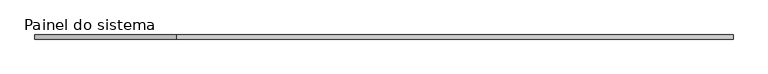
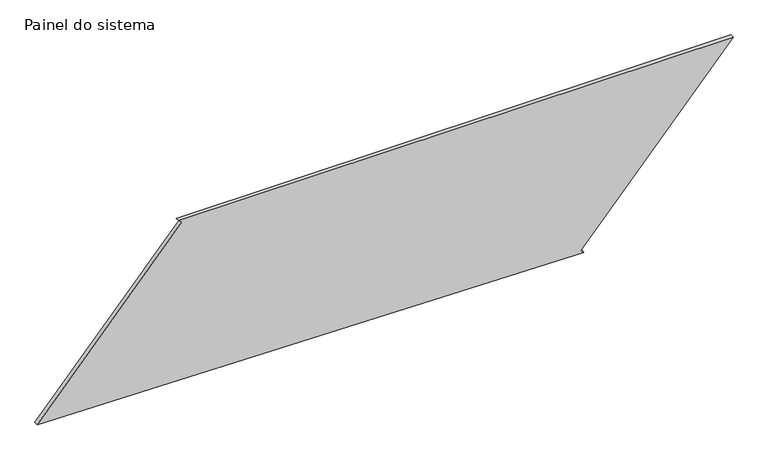
"""IFC4 building model written with IfcOpenShell, lengths in millimetres: plate geometry, Painel do sistema : Envidraçado."""

from ifc_helpers import new_model, si_unit, frame, origin, place, context, project, spatial, polyline, outline, extrude, source, transform, mapped, element, save


def painel_do_sistema_9e2e3e45(model_context):
    return source(origin(), model_context, "Body", "SweptSolid", [
        extrude(outline(polyline([(0.0, 1217.150078), (16.5356636, 1198.3998293), (1073.9840407, 2130.9533607), (1073.9840407, -1265.8401605), (1057.4483771, -1247.0899117), (55.2110382, -2130.9533607), (0.0, 1217.150078)])), frame((0.0, 24.5, 0.0), z_axis=(0.0, 1.0, 0.0), x_axis=(0.0, 0.0, 1.0)), (0.0, 0.0, 1.0), 25.0),
    ])


if __name__ == "__main__":
    model = new_model("IFC4")
    model_context = context("Model", 3, world=origin())
    ifc_project = project(units=[si_unit("LENGTHUNIT", "METRE", prefix="MILLI")], contexts=[model_context])
    site = spatial("IfcSite", under=ifc_project)
    building = spatial("IfcBuilding", under=site)
    placement = place(None, origin())
    painel_do_sistema_shape = painel_do_sistema_9e2e3e45(model_context)
    element("IfcPlate", 1, ObjectType="Painel do sistema : Envidraçado", at=placement, inside=building, context=model_context, shape_type="MappedRepresentation", body=[
        mapped(painel_do_sistema_shape, transform((0.0, 0.0, 0.0), x_axis=(1.0, 0.0, 0.0), y_axis=(0.0, 1.0, 0.0), z_axis=(0.0, 0.0, 1.0))),
    ])
    save(model, "model.ifc")

# Revit data of these elements
# Type "Painel do sistema : Envidraçado"
#   Construction Type Id = "GSP4R"
#   Analytic Construction = "Vidraça única Pilkington 1/8 pol"
#   Visual Light Transmittance = 0.9
#   Solar Heat Gain Coefficient = 0.86
#   Heat Transfer Coefficient (U) = 6.7069 W/(m²·K)
# Element 1 (IfcPlate, "Painel do sistema : Envidraçado")
#   Materials on its faces: "Vidro"
# Materials
#   "Vidro": class "Vidro", colour RGB 0 128 192, transparency 0.9, Description = "Vidro de sílica", Cost = 0
